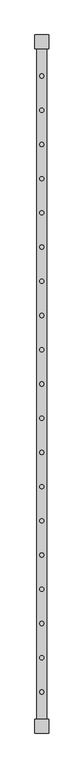
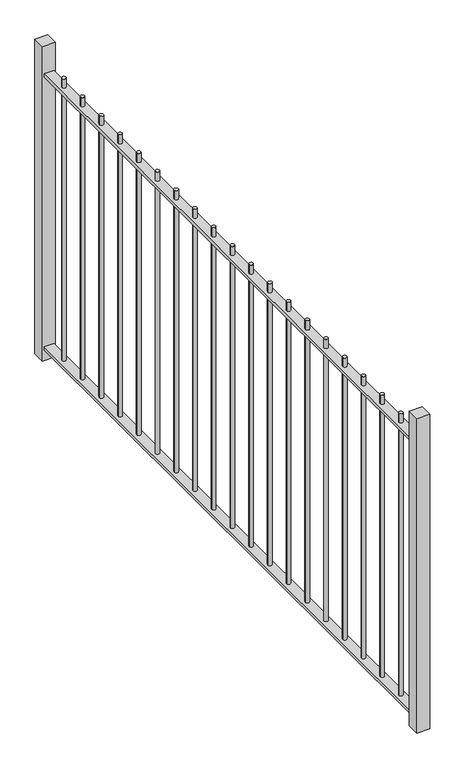
"""IFC4 building model written with IfcOpenShell, lengths in millimetres: railing geometry."""

import ifcopenshell
import ifcopenshell.guid

model = None  # the IFC model being written
_history = None  # IfcOwnerHistory: only IFC2X3 demands one
_inside = {}  # id of a spatial element -> (the spatial element, [elements in it])
_under = {}  # id of a project, library or spatial element -> (it, [spatial elements below it])
_declared = {}  # id of a project -> (the project, [libraries it declares])
_typed = {}  # id of a type object -> (the type object, [elements of that type])
_made_of = {}  # id of a material, layer set ... -> (it, [elements and type objects made of it])


def new_model(schema):
    """Start an empty IFC model of exactly this schema.

    Asked for "IFC4X3", IfcOpenShell would pick the latest addendum, in which some entities
    have other attributes; the version numbers below select the first issue.
    IFC2X3 requires an IfcOwnerHistory on every rooted entity: one is made here for all.
    """
    global model, _history
    if schema == "IFC4X3":
        model = ifcopenshell.file(schema_version=(4, 3, 0, 0))
    else:
        model = ifcopenshell.file(schema=schema)
    _inside.clear()
    _under.clear()
    _declared.clear()
    _typed.clear()
    _made_of.clear()
    _history = None
    if model.schema == "IFC2X3":
        org = make("IfcOrganization", Name="unknown")
        user = make(
            "IfcPersonAndOrganization",
            ThePerson=make("IfcPerson", FamilyName="unknown"),
            TheOrganization=org,
        )
        app = make(
            "IfcApplication",
            ApplicationDeveloper=org,
            Version="unknown",
            ApplicationFullName="unknown",
            ApplicationIdentifier="unknown",
        )
        _history = make(
            "IfcOwnerHistory",
            OwningUser=user,
            OwningApplication=app,
            ChangeAction="ADDED",
            CreationDate=0,
        )
    return model


def make(cls, **values):
    """One entity of the class cls with the attributes given. An attribute that is None is left unset."""
    return model.create_entity(
        cls, **{name: value for name, value in values.items() if value is not None}
    )


def rooted(cls, **values):
    """An entity with a GlobalId (a new one), such as an element, a storey or a relation."""
    return make(cls, GlobalId=ifcopenshell.guid.new(), OwnerHistory=_history, **values)


def si_unit(unit_type, name, prefix=None):
    """IfcSIUnit, for example si_unit("LENGTHUNIT", "METRE", prefix="MILLI")."""
    return make("IfcSIUnit", UnitType=unit_type, Prefix=prefix, Name=name)


def assignment(units):
    """IfcUnitAssignment: the units of a project."""
    return None if units is None else make("IfcUnitAssignment", Units=units)


def point(xyz):
    """IfcCartesianPoint."""
    return None if xyz is None else make("IfcCartesianPoint", Coordinates=xyz)


def direction(xyz):
    """IfcDirection."""
    return None if xyz is None else make("IfcDirection", DirectionRatios=xyz)


def frame(location, z_axis=None, x_axis=None):
    """IfcAxis2Placement3D, a coordinate frame: its origin and axes. An axis left out is left unset."""
    return make(
        "IfcAxis2Placement3D",
        Location=point(location),
        Axis=direction(z_axis),
        RefDirection=direction(x_axis),
    )


def frame_2d(location, x_axis=None):
    """IfcAxis2Placement2D, a coordinate frame in the plane: its origin and x axis."""
    return make(
        "IfcAxis2Placement2D", Location=point(location), RefDirection=direction(x_axis)
    )


def origin():
    """The frame at (0, 0, 0) with its axes left unset."""
    return frame((0.0, 0.0, 0.0))


def place(relative_to, where):
    """IfcLocalPlacement: puts the frame where relative to a parent placement (None: the world)."""
    return make(
        "IfcLocalPlacement", PlacementRelTo=relative_to, RelativePlacement=where
    )


def context(
    kind, dimensions, precision=None, world=None, true_north=None, identifier=None
):
    """IfcGeometricRepresentationContext, for example the 3D "Model" context."""
    return make(
        "IfcGeometricRepresentationContext",
        ContextIdentifier=identifier,
        ContextType=kind,
        CoordinateSpaceDimension=dimensions,
        Precision=precision,
        WorldCoordinateSystem=world,
        TrueNorth=true_north,
    )


def project(units=None, contexts=None):
    """IfcProject with its units and contexts."""
    return rooted(
        "IfcProject",
        Name="project",
        RepresentationContexts=contexts,
        UnitsInContext=assignment(units),
    )


def spatial(cls, under=None, at=None, **own):
    """A site, building, storey or space (cls), placed at a placement, below another one or the project."""
    s = rooted(cls, ObjectPlacement=at, **own)
    if under is not None:
        _under.setdefault(under.id(), (under, []))[1].append(s)
    return s


def polyline(points):
    """IfcPolyline through the points."""
    return make("IfcPolyline", Points=[point(p) for p in points])


def circle_curve(where, radius):
    """IfcCircle in the frame where."""
    return make("IfcCircle", Position=where, Radius=radius)


def trimmed(basis, trim1, trim2, sense, master):
    """IfcTrimmedCurve: the piece of a basis curve between two trims."""
    return make(
        "IfcTrimmedCurve",
        BasisCurve=basis,
        Trim1=trim1,
        Trim2=trim2,
        SenseAgreement=sense,
        MasterRepresentation=master,
    )


def segment(curve, same_sense, transition):
    """IfcCompositeCurveSegment."""
    return make(
        "IfcCompositeCurveSegment",
        Transition=transition,
        SameSense=same_sense,
        ParentCurve=curve,
    )


def composite_curve(segments, self_intersect=None):
    """IfcCompositeCurve: segments joined end to end."""
    return make("IfcCompositeCurve", Segments=segments, SelfIntersect=self_intersect)


def outline(outer, holes=None, kind="AREA"):
    """IfcArbitraryClosedProfileDef: a profile drawn as a closed curve; with holes, ...WithVoids."""
    if holes is None:
        return make("IfcArbitraryClosedProfileDef", ProfileType=kind, OuterCurve=outer)
    return make(
        "IfcArbitraryProfileDefWithVoids",
        ProfileType=kind,
        OuterCurve=outer,
        InnerCurves=holes,
    )


def extrude(swept, where, along, depth):
    """IfcExtrudedAreaSolid: the profile swept, set in the frame where, extruded along a direction by depth."""
    return make(
        "IfcExtrudedAreaSolid",
        SweptArea=swept,
        Position=where,
        ExtrudedDirection=direction(along),
        Depth=depth,
    )


def shape(context_of_items, identifier, shape_type, items):
    """IfcShapeRepresentation: the items that make up one representation, for example the "Body"."""
    return make(
        "IfcShapeRepresentation",
        ContextOfItems=context_of_items,
        RepresentationIdentifier=identifier,
        RepresentationType=shape_type,
        Items=items,
    )


def source(mapping_origin, context_of_items, identifier, shape_type, items):
    """IfcRepresentationMap: a shape defined once, which mapped items show again and again."""
    return make(
        "IfcRepresentationMap",
        MappingOrigin=mapping_origin,
        MappedRepresentation=shape(context_of_items, identifier, shape_type, items),
    )


def transform(
    local_origin,
    x_axis=None,
    y_axis=None,
    z_axis=None,
    scale=None,
    scale2=None,
    scale3=None,
    uniform=True,
):
    """IfcCartesianTransformationOperator3D, or its non-uniform kind. x_axis, y_axis, z_axis: its Axis1, 2, 3."""
    if uniform:
        return make(
            "IfcCartesianTransformationOperator3D",
            Axis1=direction(x_axis),
            Axis2=direction(y_axis),
            LocalOrigin=point(local_origin),
            Scale=scale,
            Axis3=direction(z_axis),
        )
    return make(
        "IfcCartesianTransformationOperator3DnonUniform",
        Axis1=direction(x_axis),
        Axis2=direction(y_axis),
        LocalOrigin=point(local_origin),
        Scale=scale,
        Axis3=direction(z_axis),
        Scale2=scale2,
        Scale3=scale3,
    )


def mapped(mapping_source, mapping_target):
    """IfcMappedItem: shows the shape of a source again, moved by a transform."""
    return make(
        "IfcMappedItem", MappingSource=mapping_source, MappingTarget=mapping_target
    )


def made_of(thing, what):
    """Note that an element or type object is made of a material, layer set ...; save() writes the relation."""
    if what is not None:
        _made_of.setdefault(what.id(), (what, []))[1].append(thing)
    return thing


def element(
    cls,
    number,
    at=None,
    inside=None,
    cuts=None,
    type_object=None,
    material=None,
    context=None,
    identifier="Body",
    shape_type=None,
    held_by="IfcProductDefinitionShape",
    body=None,
    shapes=None,
    **own,
):
    """One element of the class cls, such as IfcWall. Its Tag is "e" and its number.

    at: its placement. inside: the storey or other place that contains it. cuts: it is an
    opening in that element (IfcRelVoidsElement). A single representation is given by context,
    identifier, shape_type and body (its items); several are given by shapes. held_by: the class
    of the entity that holds the representations. save() writes the other relations.
    """
    e = rooted(cls, Tag="e%d" % number, ObjectPlacement=at, **own)
    if body is not None:
        shapes = [shape(context, identifier, shape_type, body)]
    if shapes is not None:
        e.Representation = make(held_by, Representations=shapes)
    if inside is not None:
        _inside.setdefault(inside.id(), (inside, []))[1].append(e)
    if cuts is not None:
        rooted(
            "IfcRelVoidsElement", RelatingBuildingElement=cuts, RelatedOpeningElement=e
        )
    if type_object is not None:
        _typed.setdefault(type_object.id(), (type_object, []))[1].append(e)
    return made_of(e, material)


def aggregate(whole, parts):
    """IfcRelAggregates: a whole, such as a stair, and the parts it consists of."""
    return rooted("IfcRelAggregates", RelatingObject=whole, RelatedObjects=parts)


def save(model, path):
    """Write the relations noted so far, then the file.

    IfcRelAggregates (storeys below a building ...), IfcRelContainedInSpatialStructure (elements
    in a storey), IfcRelDefinesByType, IfcRelAssociatesMaterial and IfcRelDeclares: one each for
    every whole, place, type object, material and project.
    """
    for whole, parts in _under.values():
        aggregate(whole, parts)
    for where, things in _inside.values():
        rooted(
            "IfcRelContainedInSpatialStructure",
            RelatedElements=things,
            RelatingStructure=where,
        )
    for kind, things in _typed.values():
        rooted("IfcRelDefinesByType", RelatedObjects=things, RelatingType=kind)
    for what, things in _made_of.values():
        rooted("IfcRelAssociatesMaterial", RelatedObjects=things, RelatingMaterial=what)
    for by, libraries in _declared.values():
        rooted("IfcRelDeclares", RelatingContext=by, RelatedDefinitions=libraries)
    model.write(path)


def railing_b46db76b(model_context):
    return source(origin(), model_context, "Body", "SweptSolid", [
        extrude(outline(polyline([(89850.4300877, 84148.8903436), (89790.4300877, 84148.8903436), (89790.4300877, 88148.8903436), (89850.4300877, 88148.8903436), (89850.4300877, 84148.8903436)])), frame((0.0, 0.0, -30.0), z_axis=(0.0, 0.0, 1.0), x_axis=(1.0, 0.0, 0.0)), (0.0, 0.0, 1.0), 20.0),
        extrude(outline(polyline([(89850.4300877, 84148.8903436), (89790.4300877, 84148.8903436), (89790.4300877, 88148.8903436), (89850.4300877, 88148.8903436), (89850.4300877, 84148.8903436)])), frame((0.0, 0.0, 1750.0), z_axis=(0.0, 0.0, 1.0), x_axis=(1.0, 0.0, 0.0)), (0.0, 0.0, 1.0), 20.0),
        extrude(outline(composite_curve([segment(trimmed(circle_curve(frame_2d((89820.4300877, 87948.8903436)), 12.5), [point((89832.9300877, 87948.8903436))], [point((89807.9300877, 87948.8903436))], False, "CARTESIAN"), True, "CONTINUOUS"), segment(trimmed(circle_curve(frame_2d((89820.4300877, 87948.8903436)), 12.5), [point((89807.9300877, 87948.8903436))], [point((89832.9300877, 87948.8903436))], False, "CARTESIAN"), True, "CONTINUOUS")], self_intersect=False)), frame((0.0, 0.0, -10.0), z_axis=(0.0, 0.0, 1.0), x_axis=(1.0, 0.0, 0.0)), (0.0, 0.0, 1.0), 1840.0),
        extrude(outline(composite_curve([segment(trimmed(circle_curve(frame_2d((89820.4300877, 87748.8903436)), 12.5), [point((89832.9300877, 87748.8903436))], [point((89807.9300877, 87748.8903436))], False, "CARTESIAN"), True, "CONTINUOUS"), segment(trimmed(circle_curve(frame_2d((89820.4300877, 87748.8903436)), 12.5), [point((89807.9300877, 87748.8903436))], [point((89832.9300877, 87748.8903436))], False, "CARTESIAN"), True, "CONTINUOUS")], self_intersect=False)), frame((0.0, 0.0, -10.0), z_axis=(0.0, 0.0, 1.0), x_axis=(1.0, 0.0, 0.0)), (0.0, 0.0, 1.0), 1840.0),
        extrude(outline(composite_curve([segment(trimmed(circle_curve(frame_2d((89820.4300877, 87548.8903436)), 12.5), [point((89832.9300877, 87548.8903436))], [point((89807.9300877, 87548.8903436))], False, "CARTESIAN"), True, "CONTINUOUS"), segment(trimmed(circle_curve(frame_2d((89820.4300877, 87548.8903436)), 12.5), [point((89807.9300877, 87548.8903436))], [point((89832.9300877, 87548.8903436))], False, "CARTESIAN"), True, "CONTINUOUS")], self_intersect=False)), frame((0.0, 0.0, -10.0), z_axis=(0.0, 0.0, 1.0), x_axis=(1.0, 0.0, 0.0)), (0.0, 0.0, 1.0), 1840.0),
        extrude(outline(composite_curve([segment(trimmed(circle_curve(frame_2d((89820.4300877, 87348.8903436)), 12.5), [point((89832.9300877, 87348.8903436))], [point((89807.9300877, 87348.8903436))], False, "CARTESIAN"), True, "CONTINUOUS"), segment(trimmed(circle_curve(frame_2d((89820.4300877, 87348.8903436)), 12.5), [point((89807.9300877, 87348.8903436))], [point((89832.9300877, 87348.8903436))], False, "CARTESIAN"), True, "CONTINUOUS")], self_intersect=False)), frame((0.0, 0.0, -10.0), z_axis=(0.0, 0.0, 1.0), x_axis=(1.0, 0.0, 0.0)), (0.0, 0.0, 1.0), 1840.0),
        extrude(outline(composite_curve([segment(trimmed(circle_curve(frame_2d((89820.4300877, 87148.8903436)), 12.5), [point((89832.9300877, 87148.8903436))], [point((89807.9300877, 87148.8903436))], False, "CARTESIAN"), True, "CONTINUOUS"), segment(trimmed(circle_curve(frame_2d((89820.4300877, 87148.8903436)), 12.5), [point((89807.9300877, 87148.8903436))], [point((89832.9300877, 87148.8903436))], False, "CARTESIAN"), True, "CONTINUOUS")], self_intersect=False)), frame((0.0, 0.0, -10.0), z_axis=(0.0, 0.0, 1.0), x_axis=(1.0, 0.0, 0.0)), (0.0, 0.0, 1.0), 1840.0),
        extrude(outline(composite_curve([segment(trimmed(circle_curve(frame_2d((89820.4300877, 86948.8903436)), 12.5), [point((89832.9300877, 86948.8903436))], [point((89807.9300877, 86948.8903436))], False, "CARTESIAN"), True, "CONTINUOUS"), segment(trimmed(circle_curve(frame_2d((89820.4300877, 86948.8903436)), 12.5), [point((89807.9300877, 86948.8903436))], [point((89832.9300877, 86948.8903436))], False, "CARTESIAN"), True, "CONTINUOUS")], self_intersect=False)), frame((0.0, 0.0, -10.0), z_axis=(0.0, 0.0, 1.0), x_axis=(1.0, 0.0, 0.0)), (0.0, 0.0, 1.0), 1840.0),
        extrude(outline(composite_curve([segment(trimmed(circle_curve(frame_2d((89820.4300877, 86748.8903436)), 12.5), [point((89832.9300877, 86748.8903436))], [point((89807.9300877, 86748.8903436))], False, "CARTESIAN"), True, "CONTINUOUS"), segment(trimmed(circle_curve(frame_2d((89820.4300877, 86748.8903436)), 12.5), [point((89807.9300877, 86748.8903436))], [point((89832.9300877, 86748.8903436))], False, "CARTESIAN"), True, "CONTINUOUS")], self_intersect=False)), frame((0.0, 0.0, -10.0), z_axis=(0.0, 0.0, 1.0), x_axis=(1.0, 0.0, 0.0)), (0.0, 0.0, 1.0), 1840.0),
        extrude(outline(composite_curve([segment(trimmed(circle_curve(frame_2d((89820.4300877, 86548.8903436)), 12.5), [point((89832.9300877, 86548.8903436))], [point((89807.9300877, 86548.8903436))], False, "CARTESIAN"), True, "CONTINUOUS"), segment(trimmed(circle_curve(frame_2d((89820.4300877, 86548.8903436)), 12.5), [point((89807.9300877, 86548.8903436))], [point((89832.9300877, 86548.8903436))], False, "CARTESIAN"), True, "CONTINUOUS")], self_intersect=False)), frame((0.0, 0.0, -10.0), z_axis=(0.0, 0.0, 1.0), x_axis=(1.0, 0.0, 0.0)), (0.0, 0.0, 1.0), 1840.0),
        extrude(outline(composite_curve([segment(trimmed(circle_curve(frame_2d((89820.4300877, 86348.8903436)), 12.5), [point((89832.9300877, 86348.8903436))], [point((89807.9300877, 86348.8903436))], False, "CARTESIAN"), True, "CONTINUOUS"), segment(trimmed(circle_curve(frame_2d((89820.4300877, 86348.8903436)), 12.5), [point((89807.9300877, 86348.8903436))], [point((89832.9300877, 86348.8903436))], False, "CARTESIAN"), True, "CONTINUOUS")], self_intersect=False)), frame((0.0, 0.0, -10.0), z_axis=(0.0, 0.0, 1.0), x_axis=(1.0, 0.0, 0.0)), (0.0, 0.0, 1.0), 1840.0),
        extrude(outline(composite_curve([segment(trimmed(circle_curve(frame_2d((89820.4300877, 86148.8903436)), 12.5), [point((89832.9300877, 86148.8903436))], [point((89807.9300877, 86148.8903436))], False, "CARTESIAN"), True, "CONTINUOUS"), segment(trimmed(circle_curve(frame_2d((89820.4300877, 86148.8903436)), 12.5), [point((89807.9300877, 86148.8903436))], [point((89832.9300877, 86148.8903436))], False, "CARTESIAN"), True, "CONTINUOUS")], self_intersect=False)), frame((0.0, 0.0, -10.0), z_axis=(0.0, 0.0, 1.0), x_axis=(1.0, 0.0, 0.0)), (0.0, 0.0, 1.0), 1840.0),
        extrude(outline(composite_curve([segment(trimmed(circle_curve(frame_2d((89820.4300877, 85948.8903436)), 12.5), [point((89832.9300877, 85948.8903436))], [point((89807.9300877, 85948.8903436))], False, "CARTESIAN"), True, "CONTINUOUS"), segment(trimmed(circle_curve(frame_2d((89820.4300877, 85948.8903436)), 12.5), [point((89807.9300877, 85948.8903436))], [point((89832.9300877, 85948.8903436))], False, "CARTESIAN"), True, "CONTINUOUS")], self_intersect=False)), frame((0.0, 0.0, -10.0), z_axis=(0.0, 0.0, 1.0), x_axis=(1.0, 0.0, 0.0)), (0.0, 0.0, 1.0), 1840.0),
        extrude(outline(composite_curve([segment(trimmed(circle_curve(frame_2d((89820.4300877, 85748.8903436)), 12.5), [point((89832.9300877, 85748.8903436))], [point((89807.9300877, 85748.8903436))], False, "CARTESIAN"), True, "CONTINUOUS"), segment(trimmed(circle_curve(frame_2d((89820.4300877, 85748.8903436)), 12.5), [point((89807.9300877, 85748.8903436))], [point((89832.9300877, 85748.8903436))], False, "CARTESIAN"), True, "CONTINUOUS")], self_intersect=False)), frame((0.0, 0.0, -10.0), z_axis=(0.0, 0.0, 1.0), x_axis=(1.0, 0.0, 0.0)), (0.0, 0.0, 1.0), 1840.0),
        extrude(outline(composite_curve([segment(trimmed(circle_curve(frame_2d((89820.4300877, 85548.8903436)), 12.5), [point((89832.9300877, 85548.8903436))], [point((89807.9300877, 85548.8903436))], False, "CARTESIAN"), True, "CONTINUOUS"), segment(trimmed(circle_curve(frame_2d((89820.4300877, 85548.8903436)), 12.5), [point((89807.9300877, 85548.8903436))], [point((89832.9300877, 85548.8903436))], False, "CARTESIAN"), True, "CONTINUOUS")], self_intersect=False)), frame((0.0, 0.0, -10.0), z_axis=(0.0, 0.0, 1.0), x_axis=(1.0, 0.0, 0.0)), (0.0, 0.0, 1.0), 1840.0),
        extrude(outline(composite_curve([segment(trimmed(circle_curve(frame_2d((89820.4300877, 85348.8903436)), 12.5), [point((89832.9300877, 85348.8903436))], [point((89807.9300877, 85348.8903436))], False, "CARTESIAN"), True, "CONTINUOUS"), segment(trimmed(circle_curve(frame_2d((89820.4300877, 85348.8903436)), 12.5), [point((89807.9300877, 85348.8903436))], [point((89832.9300877, 85348.8903436))], False, "CARTESIAN"), True, "CONTINUOUS")], self_intersect=False)), frame((0.0, 0.0, -10.0), z_axis=(0.0, 0.0, 1.0), x_axis=(1.0, 0.0, 0.0)), (0.0, 0.0, 1.0), 1840.0),
        extrude(outline(composite_curve([segment(trimmed(circle_curve(frame_2d((89820.4300877, 85148.8903436)), 12.5), [point((89832.9300877, 85148.8903436))], [point((89807.9300877, 85148.8903436))], False, "CARTESIAN"), True, "CONTINUOUS"), segment(trimmed(circle_curve(frame_2d((89820.4300877, 85148.8903436)), 12.5), [point((89807.9300877, 85148.8903436))], [point((89832.9300877, 85148.8903436))], False, "CARTESIAN"), True, "CONTINUOUS")], self_intersect=False)), frame((0.0, 0.0, -10.0), z_axis=(0.0, 0.0, 1.0), x_axis=(1.0, 0.0, 0.0)), (0.0, 0.0, 1.0), 1840.0),
        extrude(outline(composite_curve([segment(trimmed(circle_curve(frame_2d((89820.4300877, 84948.8903436)), 12.5), [point((89832.9300877, 84948.8903436))], [point((89807.9300877, 84948.8903436))], False, "CARTESIAN"), True, "CONTINUOUS"), segment(trimmed(circle_curve(frame_2d((89820.4300877, 84948.8903436)), 12.5), [point((89807.9300877, 84948.8903436))], [point((89832.9300877, 84948.8903436))], False, "CARTESIAN"), True, "CONTINUOUS")], self_intersect=False)), frame((0.0, 0.0, -10.0), z_axis=(0.0, 0.0, 1.0), x_axis=(1.0, 0.0, 0.0)), (0.0, 0.0, 1.0), 1840.0),
        extrude(outline(composite_curve([segment(trimmed(circle_curve(frame_2d((89820.4300877, 84748.8903436)), 12.5), [point((89832.9300877, 84748.8903436))], [point((89807.9300877, 84748.8903436))], False, "CARTESIAN"), True, "CONTINUOUS"), segment(trimmed(circle_curve(frame_2d((89820.4300877, 84748.8903436)), 12.5), [point((89807.9300877, 84748.8903436))], [point((89832.9300877, 84748.8903436))], False, "CARTESIAN"), True, "CONTINUOUS")], self_intersect=False)), frame((0.0, 0.0, -10.0), z_axis=(0.0, 0.0, 1.0), x_axis=(1.0, 0.0, 0.0)), (0.0, 0.0, 1.0), 1840.0),
        extrude(outline(composite_curve([segment(trimmed(circle_curve(frame_2d((89820.4300877, 84548.8903436)), 12.5), [point((89832.9300877, 84548.8903436))], [point((89807.9300877, 84548.8903436))], False, "CARTESIAN"), True, "CONTINUOUS"), segment(trimmed(circle_curve(frame_2d((89820.4300877, 84548.8903436)), 12.5), [point((89807.9300877, 84548.8903436))], [point((89832.9300877, 84548.8903436))], False, "CARTESIAN"), True, "CONTINUOUS")], self_intersect=False)), frame((0.0, 0.0, -10.0), z_axis=(0.0, 0.0, 1.0), x_axis=(1.0, 0.0, 0.0)), (0.0, 0.0, 1.0), 1840.0),
        extrude(outline(composite_curve([segment(trimmed(circle_curve(frame_2d((89820.4300877, 84348.8903436)), 12.5), [point((89832.9300877, 84348.8903436))], [point((89807.9300877, 84348.8903436))], False, "CARTESIAN"), True, "CONTINUOUS"), segment(trimmed(circle_curve(frame_2d((89820.4300877, 84348.8903436)), 12.5), [point((89807.9300877, 84348.8903436))], [point((89832.9300877, 84348.8903436))], False, "CARTESIAN"), True, "CONTINUOUS")], self_intersect=False)), frame((0.0, 0.0, -10.0), z_axis=(0.0, 0.0, 1.0), x_axis=(1.0, 0.0, 0.0)), (0.0, 0.0, 1.0), 1840.0),
        extrude(outline(polyline([(89780.4300877, 88108.8903436), (89780.4300877, 88188.8903436), (89860.4300877, 88188.8903436), (89860.4300877, 88108.8903436), (89780.4300877, 88108.8903436)])), frame((0.0, 0.0, -100.0), z_axis=(0.0, 0.0, 1.0), x_axis=(1.0, 0.0, 0.0)), (0.0, 0.0, 1.0), 2050.0),
        extrude(outline(polyline([(89780.4300877, 84108.8903436), (89780.4300877, 84188.8903436), (89860.4300877, 84188.8903436), (89860.4300877, 84108.8903436), (89780.4300877, 84108.8903436)])), frame((0.0, 0.0, -100.0), z_axis=(0.0, 0.0, 1.0), x_axis=(1.0, 0.0, 0.0)), (0.0, 0.0, 1.0), 2050.0),
    ])


if __name__ == "__main__":
    model = new_model("IFC4")
    model_context = context("Model", 3, world=origin())
    ifc_project = project(units=[si_unit("LENGTHUNIT", "METRE", prefix="MILLI")], contexts=[model_context])
    site = spatial("IfcSite", under=ifc_project)
    building = spatial("IfcBuilding", under=site)
    placement = place(None, origin())
    railing_shape = railing_b46db76b(model_context)
    element("IfcRailing", 1, at=placement, inside=building, context=model_context, shape_type="MappedRepresentation", body=[
        mapped(railing_shape, transform((0.0, 0.0, 0.0), x_axis=(1.0, 0.0, 0.0), y_axis=(0.0, 1.0, 0.0), z_axis=(0.0, 0.0, 1.0))),
    ])
    save(model, "model.ifc")

# Revit data of these elements
# Element 1 (IfcRailing)
#   Materials on its faces: "NLRS_h2_staal_generiek zwart_gen_rsf", "NLRS_h2_staal_gen_rsf"
# Materials
#   "NLRS_h2_staal_generiek zwart_gen_rsf": class "Metal", colour RGB 189 187 185, transparency 0, Manufacturer = "RevitGG", URL = "www.revitgg.nl", Description = "Staal, generiek materiaal", Cost = 0
#   "NLRS_h2_staal_gen_rsf": class "H - Metaal", colour RGB 189 187 185, transparency 0, Keynote = "h2", Model = "generiek", Manufacturer = "Revit Standards Foundation", URL = "www.revitstandards.org", Description = "staal", Cost = 0
